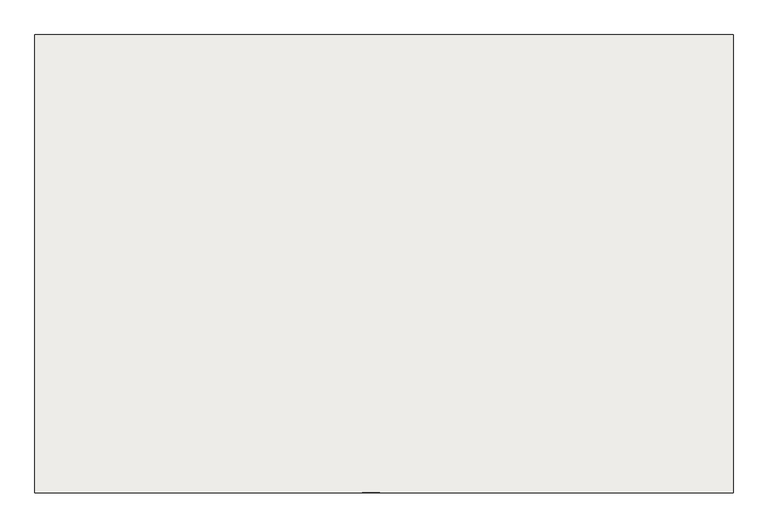
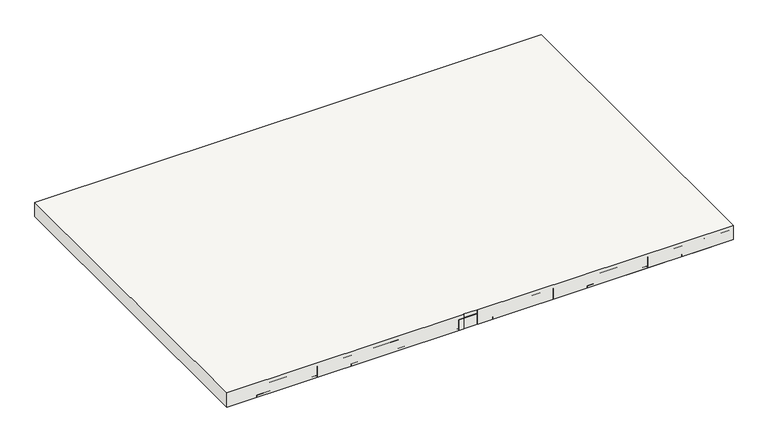
"""IFC4 building model written with IfcOpenShell, lengths in millimetres: slab geometry, Pano 2 (16 cm)."""

import ifcopenshell
import ifcopenshell.guid

model = None  # the IFC model being written
_history = None  # IfcOwnerHistory: only IFC2X3 demands one
_inside = {}  # id of a spatial element -> (the spatial element, [elements in it])
_under = {}  # id of a project, library or spatial element -> (it, [spatial elements below it])
_declared = {}  # id of a project -> (the project, [libraries it declares])
_typed = {}  # id of a type object -> (the type object, [elements of that type])
_made_of = {}  # id of a material, layer set ... -> (it, [elements and type objects made of it])


def new_model(schema):
    """Start an empty IFC model of exactly this schema.

    Asked for "IFC4X3", IfcOpenShell would pick the latest addendum, in which some entities
    have other attributes; the version numbers below select the first issue.
    IFC2X3 requires an IfcOwnerHistory on every rooted entity: one is made here for all.
    """
    global model, _history
    if schema == "IFC4X3":
        model = ifcopenshell.file(schema_version=(4, 3, 0, 0))
    else:
        model = ifcopenshell.file(schema=schema)
    _inside.clear()
    _under.clear()
    _declared.clear()
    _typed.clear()
    _made_of.clear()
    _history = None
    if model.schema == "IFC2X3":
        org = make("IfcOrganization", Name="unknown")
        user = make(
            "IfcPersonAndOrganization",
            ThePerson=make("IfcPerson", FamilyName="unknown"),
            TheOrganization=org,
        )
        app = make(
            "IfcApplication",
            ApplicationDeveloper=org,
            Version="unknown",
            ApplicationFullName="unknown",
            ApplicationIdentifier="unknown",
        )
        _history = make(
            "IfcOwnerHistory",
            OwningUser=user,
            OwningApplication=app,
            ChangeAction="ADDED",
            CreationDate=0,
        )
    return model


def make(cls, **values):
    """One entity of the class cls with the attributes given. An attribute that is None is left unset."""
    return model.create_entity(
        cls, **{name: value for name, value in values.items() if value is not None}
    )


def rooted(cls, **values):
    """An entity with a GlobalId (a new one), such as an element, a storey or a relation."""
    return make(cls, GlobalId=ifcopenshell.guid.new(), OwnerHistory=_history, **values)


def si_unit(unit_type, name, prefix=None):
    """IfcSIUnit, for example si_unit("LENGTHUNIT", "METRE", prefix="MILLI")."""
    return make("IfcSIUnit", UnitType=unit_type, Prefix=prefix, Name=name)


def assignment(units):
    """IfcUnitAssignment: the units of a project."""
    return None if units is None else make("IfcUnitAssignment", Units=units)


def point(xyz):
    """IfcCartesianPoint."""
    return None if xyz is None else make("IfcCartesianPoint", Coordinates=xyz)


def direction(xyz):
    """IfcDirection."""
    return None if xyz is None else make("IfcDirection", DirectionRatios=xyz)


def frame(location, z_axis=None, x_axis=None):
    """IfcAxis2Placement3D, a coordinate frame: its origin and axes. An axis left out is left unset."""
    return make(
        "IfcAxis2Placement3D",
        Location=point(location),
        Axis=direction(z_axis),
        RefDirection=direction(x_axis),
    )


def origin():
    """The frame at (0, 0, 0) with its axes left unset."""
    return frame((0.0, 0.0, 0.0))


def origin_with_axes():
    """The frame at (0, 0, 0) with the z axis (0, 0, 1) and the x axis (1, 0, 0) written out."""
    return frame((0.0, 0.0, 0.0), z_axis=(0.0, 0.0, 1.0), x_axis=(1.0, 0.0, 0.0))


def place(relative_to, where):
    """IfcLocalPlacement: puts the frame where relative to a parent placement (None: the world)."""
    return make(
        "IfcLocalPlacement", PlacementRelTo=relative_to, RelativePlacement=where
    )


def context(
    kind, dimensions, precision=None, world=None, true_north=None, identifier=None
):
    """IfcGeometricRepresentationContext, for example the 3D "Model" context."""
    return make(
        "IfcGeometricRepresentationContext",
        ContextIdentifier=identifier,
        ContextType=kind,
        CoordinateSpaceDimension=dimensions,
        Precision=precision,
        WorldCoordinateSystem=world,
        TrueNorth=true_north,
    )


def project(units=None, contexts=None):
    """IfcProject with its units and contexts."""
    return rooted(
        "IfcProject",
        Name="project",
        RepresentationContexts=contexts,
        UnitsInContext=assignment(units),
    )


def spatial(cls, under=None, at=None, **own):
    """A site, building, storey or space (cls), placed at a placement, below another one or the project."""
    s = rooted(cls, ObjectPlacement=at, **own)
    if under is not None:
        _under.setdefault(under.id(), (under, []))[1].append(s)
    return s


def polyline(points):
    """IfcPolyline through the points."""
    return make("IfcPolyline", Points=[point(p) for p in points])


def outline(outer, holes=None, kind="AREA"):
    """IfcArbitraryClosedProfileDef: a profile drawn as a closed curve; with holes, ...WithVoids."""
    if holes is None:
        return make("IfcArbitraryClosedProfileDef", ProfileType=kind, OuterCurve=outer)
    return make(
        "IfcArbitraryProfileDefWithVoids",
        ProfileType=kind,
        OuterCurve=outer,
        InnerCurves=holes,
    )


def extrude(swept, where, along, depth):
    """IfcExtrudedAreaSolid: the profile swept, set in the frame where, extruded along a direction by depth."""
    return make(
        "IfcExtrudedAreaSolid",
        SweptArea=swept,
        Position=where,
        ExtrudedDirection=direction(along),
        Depth=depth,
    )


def shape(context_of_items, identifier, shape_type, items):
    """IfcShapeRepresentation: the items that make up one representation, for example the "Body"."""
    return make(
        "IfcShapeRepresentation",
        ContextOfItems=context_of_items,
        RepresentationIdentifier=identifier,
        RepresentationType=shape_type,
        Items=items,
    )


def source(mapping_origin, context_of_items, identifier, shape_type, items):
    """IfcRepresentationMap: a shape defined once, which mapped items show again and again."""
    return make(
        "IfcRepresentationMap",
        MappingOrigin=mapping_origin,
        MappedRepresentation=shape(context_of_items, identifier, shape_type, items),
    )


def transform(
    local_origin,
    x_axis=None,
    y_axis=None,
    z_axis=None,
    scale=None,
    scale2=None,
    scale3=None,
    uniform=True,
):
    """IfcCartesianTransformationOperator3D, or its non-uniform kind. x_axis, y_axis, z_axis: its Axis1, 2, 3."""
    if uniform:
        return make(
            "IfcCartesianTransformationOperator3D",
            Axis1=direction(x_axis),
            Axis2=direction(y_axis),
            LocalOrigin=point(local_origin),
            Scale=scale,
            Axis3=direction(z_axis),
        )
    return make(
        "IfcCartesianTransformationOperator3DnonUniform",
        Axis1=direction(x_axis),
        Axis2=direction(y_axis),
        LocalOrigin=point(local_origin),
        Scale=scale,
        Axis3=direction(z_axis),
        Scale2=scale2,
        Scale3=scale3,
    )


def mapped(mapping_source, mapping_target):
    """IfcMappedItem: shows the shape of a source again, moved by a transform."""
    return make(
        "IfcMappedItem", MappingSource=mapping_source, MappingTarget=mapping_target
    )


def made_of(thing, what):
    """Note that an element or type object is made of a material, layer set ...; save() writes the relation."""
    if what is not None:
        _made_of.setdefault(what.id(), (what, []))[1].append(thing)
    return thing


def element(
    cls,
    number,
    at=None,
    inside=None,
    cuts=None,
    type_object=None,
    material=None,
    context=None,
    identifier="Body",
    shape_type=None,
    held_by="IfcProductDefinitionShape",
    body=None,
    shapes=None,
    **own,
):
    """One element of the class cls, such as IfcWall. Its Tag is "e" and its number.

    at: its placement. inside: the storey or other place that contains it. cuts: it is an
    opening in that element (IfcRelVoidsElement). A single representation is given by context,
    identifier, shape_type and body (its items); several are given by shapes. held_by: the class
    of the entity that holds the representations. save() writes the other relations.
    """
    e = rooted(cls, Tag="e%d" % number, ObjectPlacement=at, **own)
    if body is not None:
        shapes = [shape(context, identifier, shape_type, body)]
    if shapes is not None:
        e.Representation = make(held_by, Representations=shapes)
    if inside is not None:
        _inside.setdefault(inside.id(), (inside, []))[1].append(e)
    if cuts is not None:
        rooted(
            "IfcRelVoidsElement", RelatingBuildingElement=cuts, RelatedOpeningElement=e
        )
    if type_object is not None:
        _typed.setdefault(type_object.id(), (type_object, []))[1].append(e)
    return made_of(e, material)


def aggregate(whole, parts):
    """IfcRelAggregates: a whole, such as a stair, and the parts it consists of."""
    return rooted("IfcRelAggregates", RelatingObject=whole, RelatedObjects=parts)


def save(model, path):
    """Write the relations noted so far, then the file.

    IfcRelAggregates (storeys below a building ...), IfcRelContainedInSpatialStructure (elements
    in a storey), IfcRelDefinesByType, IfcRelAssociatesMaterial and IfcRelDeclares: one each for
    every whole, place, type object, material and project.
    """
    for whole, parts in _under.values():
        aggregate(whole, parts)
    for where, things in _inside.values():
        rooted(
            "IfcRelContainedInSpatialStructure",
            RelatedElements=things,
            RelatingStructure=where,
        )
    for kind, things in _typed.values():
        rooted("IfcRelDefinesByType", RelatedObjects=things, RelatingType=kind)
    for what, things in _made_of.values():
        rooted("IfcRelAssociatesMaterial", RelatedObjects=things, RelatingMaterial=what)
    for by, libraries in _declared.values():
        rooted("IfcRelDeclares", RelatingContext=by, RelatedDefinitions=libraries)
    model.write(path)


def slab_4fb4e0ab(model_context):
    return source(origin(), model_context, "Body", "SweptSolid", [
        extrude(outline(polyline([(-1000.0, 6010.0), (-1000.0, 2490.0), (-3710.0, 2490.0), (-3710.0, 2495.0), (-3850.0, 2495.0), (-3850.0, 2490.0), (-6360.0, 2490.0), (-6360.0, 6010.0), (-1000.0, 6010.0)])), origin_with_axes(), (0.0, 0.0, 1.0), 160.0),
        extrude(outline(polyline([(-5045.0, 5490.0), (-5405.0, 5490.0), (-5405.0, 5985.0), (-5045.0, 5985.0), (-5045.0, 5490.0)])), origin_with_axes(), (0.0, 0.0, 1.0), 120.0),
        extrude(outline(polyline([(-1545.0, 3990.0), (-1905.0, 3990.0), (-1905.0, 4485.0), (-1545.0, 4485.0), (-1545.0, 3990.0)])), origin_with_axes(), (0.0, 0.0, 1.0), 120.0),
        extrude(outline(polyline([(-4045.0, 4990.0), (-4405.0, 4990.0), (-4405.0, 5485.0), (-4045.0, 5485.0), (-4045.0, 4990.0)])), origin_with_axes(), (0.0, 0.0, 1.0), 120.0),
        extrude(outline(polyline([(-5545.0, 3490.0), (-5905.0, 3490.0), (-5905.0, 3985.0), (-5545.0, 3985.0), (-5545.0, 3490.0)])), origin_with_axes(), (0.0, 0.0, 1.0), 120.0),
        extrude(outline(polyline([(-2045.0, 5990.0), (-2405.0, 5990.0), (-2405.0, 6005.0), (-2045.0, 6005.0), (-2045.0, 5990.0)])), origin_with_axes(), (0.0, 0.0, 1.0), 120.0),
        extrude(outline(polyline([(-3545.0, 2490.0), (-3905.0, 2490.0), (-3905.0, 2985.0), (-3545.0, 2985.0), (-3545.0, 2490.0)])), origin_with_axes(), (0.0, 0.0, 1.0), 120.0),
        extrude(outline(polyline([(-5545.0, 2990.0), (-5905.0, 2990.0), (-5905.0, 3485.0), (-5545.0, 3485.0), (-5545.0, 2990.0)])), origin_with_axes(), (0.0, 0.0, 1.0), 120.0),
        extrude(outline(polyline([(-3905.0, 2490.0), (-4045.0, 2490.0), (-4045.0, 6010.0), (-3905.0, 6010.0), (-3905.0, 2490.0)])), origin_with_axes(), (0.0, 0.0, 1.0), 24.0),
        extrude(outline(polyline([(-5545.0, 5490.0), (-5905.0, 5490.0), (-5905.0, 5985.0), (-5545.0, 5985.0), (-5545.0, 5490.0)])), origin_with_axes(), (0.0, 0.0, 1.0), 120.0),
        extrude(outline(polyline([(-2545.0, 2990.0), (-2905.0, 2990.0), (-2905.0, 3485.0), (-2545.0, 3485.0), (-2545.0, 2990.0)])), origin_with_axes(), (0.0, 0.0, 1.0), 120.0),
        extrude(outline(polyline([(-3045.0, 5490.0), (-3405.0, 5490.0), (-3405.0, 5985.0), (-3045.0, 5985.0), (-3045.0, 5490.0)])), origin_with_axes(), (0.0, 0.0, 1.0), 120.0),
        extrude(outline(polyline([(-2045.0, 2490.0), (-2405.0, 2490.0), (-2405.0, 2985.0), (-2045.0, 2985.0), (-2045.0, 2490.0)])), origin_with_axes(), (0.0, 0.0, 1.0), 120.0),
        extrude(outline(polyline([(-4045.0, 5490.0), (-4405.0, 5490.0), (-4405.0, 5985.0), (-4045.0, 5985.0), (-4045.0, 5490.0)])), origin_with_axes(), (0.0, 0.0, 1.0), 120.0),
        extrude(outline(polyline([(-2545.0, 3490.0), (-2905.0, 3490.0), (-2905.0, 3985.0), (-2545.0, 3985.0), (-2545.0, 3490.0)])), origin_with_axes(), (0.0, 0.0, 1.0), 120.0),
        extrude(outline(polyline([(-2545.0, 2490.0), (-2905.0, 2490.0), (-2905.0, 2985.0), (-2545.0, 2985.0), (-2545.0, 2490.0)])), origin_with_axes(), (0.0, 0.0, 1.0), 120.0),
        extrude(outline(polyline([(-2545.0, 4990.0), (-2905.0, 4990.0), (-2905.0, 5485.0), (-2545.0, 5485.0), (-2545.0, 4990.0)])), origin_with_axes(), (0.0, 0.0, 1.0), 120.0),
        extrude(outline(polyline([(-3045.0, 2490.0), (-3405.0, 2490.0), (-3405.0, 2985.0), (-3045.0, 2985.0), (-3045.0, 2490.0)])), origin_with_axes(), (0.0, 0.0, 1.0), 120.0),
        extrude(outline(polyline([(-1044.5, 4990.0), (-1404.5, 4990.0), (-1404.5, 5485.0), (-1044.5, 5485.0), (-1044.5, 4990.0)])), origin_with_axes(), (0.0, 0.0, 1.0), 120.0),
        extrude(outline(polyline([(-4045.0, 2490.0), (-4405.0, 2490.0), (-4405.0, 2985.0), (-4045.0, 2985.0), (-4045.0, 2490.0)])), origin_with_axes(), (0.0, 0.0, 1.0), 120.0),
        extrude(outline(polyline([(-1545.0, 2490.0), (-1905.0, 2490.0), (-1905.0, 2985.0), (-1545.0, 2985.0), (-1545.0, 2490.0)])), origin_with_axes(), (0.0, 0.0, 1.0), 120.0),
        extrude(outline(polyline([(-2045.0, 3490.0), (-2405.0, 3490.0), (-2405.0, 3985.0), (-2045.0, 3985.0), (-2045.0, 3490.0)])), origin_with_axes(), (0.0, 0.0, 1.0), 120.0),
        extrude(outline(polyline([(-5545.0, 2490.0), (-5905.0, 2490.0), (-5905.0, 2985.0), (-5545.0, 2985.0), (-5545.0, 2490.0)])), origin_with_axes(), (0.0, 0.0, 1.0), 120.0),
        extrude(outline(polyline([(-2045.0, 5490.0), (-2405.0, 5490.0), (-2405.0, 5985.0), (-2045.0, 5985.0), (-2045.0, 5490.0)])), origin_with_axes(), (0.0, 0.0, 1.0), 120.0),
        extrude(outline(polyline([(-4545.0, 5490.0), (-4905.0, 5490.0), (-4905.0, 5985.0), (-4545.0, 5985.0), (-4545.0, 5490.0)])), origin_with_axes(), (0.0, 0.0, 1.0), 120.0),
        extrude(outline(polyline([(-2045.0, 4990.0), (-2405.0, 4990.0), (-2405.0, 5485.0), (-2045.0, 5485.0), (-2045.0, 4990.0)])), origin_with_axes(), (0.0, 0.0, 1.0), 120.0),
        extrude(outline(polyline([(-4045.0, 4490.0), (-4405.0, 4490.0), (-4405.0, 4985.0), (-4045.0, 4985.0), (-4045.0, 4490.0)])), origin_with_axes(), (0.0, 0.0, 1.0), 120.0),
        extrude(outline(polyline([(-5545.0, 3990.0), (-5905.0, 3990.0), (-5905.0, 4485.0), (-5545.0, 4485.0), (-5545.0, 3990.0)])), origin_with_axes(), (0.0, 0.0, 1.0), 120.0),
        extrude(outline(polyline([(-3045.0, 3490.0), (-3405.0, 3490.0), (-3405.0, 3985.0), (-3045.0, 3985.0), (-3045.0, 3490.0)])), origin_with_axes(), (0.0, 0.0, 1.0), 120.0),
        extrude(outline(polyline([(-3045.0, 5990.0), (-3405.0, 5990.0), (-3405.0, 6005.0), (-3045.0, 6005.0), (-3045.0, 5990.0)])), origin_with_axes(), (0.0, 0.0, 1.0), 120.0),
        extrude(outline(polyline([(-4545.0, 3490.0), (-4905.0, 3490.0), (-4905.0, 3985.0), (-4545.0, 3985.0), (-4545.0, 3490.0)])), origin_with_axes(), (0.0, 0.0, 1.0), 120.0),
        extrude(outline(polyline([(-4545.0, 5990.0), (-4905.0, 5990.0), (-4905.0, 6005.0), (-4545.0, 6005.0), (-4545.0, 5990.0)])), origin_with_axes(), (0.0, 0.0, 1.0), 120.0),
        extrude(outline(polyline([(-3045.0, 4490.0), (-3405.0, 4490.0), (-3405.0, 4985.0), (-3045.0, 4985.0), (-3045.0, 4490.0)])), origin_with_axes(), (0.0, 0.0, 1.0), 120.0),
        extrude(outline(polyline([(-4045.0, 2990.0), (-4405.0, 2990.0), (-4405.0, 3485.0), (-4045.0, 3485.0), (-4045.0, 2990.0)])), origin_with_axes(), (0.0, 0.0, 1.0), 120.0),
        extrude(outline(polyline([(-4545.0, 2490.0), (-4905.0, 2490.0), (-4905.0, 2985.0), (-4545.0, 2985.0), (-4545.0, 2490.0)])), origin_with_axes(), (0.0, 0.0, 1.0), 120.0),
        extrude(outline(polyline([(-2045.0, 3990.0), (-2405.0, 3990.0), (-2405.0, 4485.0), (-2045.0, 4485.0), (-2045.0, 3990.0)])), origin_with_axes(), (0.0, 0.0, 1.0), 120.0),
        extrude(outline(polyline([(-5045.0, 5990.0), (-5405.0, 5990.0), (-5405.0, 6005.0), (-5045.0, 6005.0), (-5045.0, 5990.0)])), origin_with_axes(), (0.0, 0.0, 1.0), 120.0),
        extrude(outline(polyline([(-2045.0, 2990.0), (-2405.0, 2990.0), (-2405.0, 3485.0), (-2045.0, 3485.0), (-2045.0, 2990.0)])), origin_with_axes(), (0.0, 0.0, 1.0), 120.0),
        extrude(outline(polyline([(-2545.0, 5990.0), (-2905.0, 5990.0), (-2905.0, 6005.0), (-2545.0, 6005.0), (-2545.0, 5990.0)])), origin_with_axes(), (0.0, 0.0, 1.0), 120.0),
        extrude(outline(polyline([(-1545.0, 4990.0), (-1905.0, 4990.0), (-1905.0, 5485.0), (-1545.0, 5485.0), (-1545.0, 4990.0)])), origin_with_axes(), (0.0, 0.0, 1.0), 120.0),
        extrude(outline(polyline([(-4045.0, 5990.0), (-4405.0, 5990.0), (-4405.0, 6005.0), (-4045.0, 6005.0), (-4045.0, 5990.0)])), origin_with_axes(), (0.0, 0.0, 1.0), 120.0),
        extrude(outline(polyline([(-2045.0, 4490.0), (-2405.0, 4490.0), (-2405.0, 4985.0), (-2045.0, 4985.0), (-2045.0, 4490.0)])), origin_with_axes(), (0.0, 0.0, 1.0), 120.0),
        extrude(outline(polyline([(-4905.0, 2490.0), (-5045.0, 2490.0), (-5045.0, 6010.0), (-4905.0, 6010.0), (-4905.0, 2490.0)])), origin_with_axes(), (0.0, 0.0, 1.0), 24.0),
        extrude(outline(polyline([(-3045.0, 3990.0), (-3405.0, 3990.0), (-3405.0, 4485.0), (-3045.0, 4485.0), (-3045.0, 3990.0)])), origin_with_axes(), (0.0, 0.0, 1.0), 120.0),
        extrude(outline(polyline([(-1545.0, 5990.0), (-1905.0, 5990.0), (-1905.0, 6005.0), (-1545.0, 6005.0), (-1545.0, 5990.0)])), origin_with_axes(), (0.0, 0.0, 1.0), 120.0),
        extrude(outline(polyline([(-3405.0, 2490.0), (-3545.0, 2490.0), (-3545.0, 6010.0), (-3405.0, 6010.0), (-3405.0, 2490.0)])), origin_with_axes(), (0.0, 0.0, 1.0), 24.0),
        extrude(outline(polyline([(-2545.0, 5490.0), (-2905.0, 5490.0), (-2905.0, 5985.0), (-2545.0, 5985.0), (-2545.0, 5490.0)])), origin_with_axes(), (0.0, 0.0, 1.0), 120.0),
        extrude(outline(polyline([(-4545.0, 2990.0), (-4905.0, 2990.0), (-4905.0, 3485.0), (-4545.0, 3485.0), (-4545.0, 2990.0)])), origin_with_axes(), (0.0, 0.0, 1.0), 120.0),
        extrude(outline(polyline([(-4045.0, 3990.0), (-4405.0, 3990.0), (-4405.0, 4485.0), (-4045.0, 4485.0), (-4045.0, 3990.0)])), origin_with_axes(), (0.0, 0.0, 1.0), 120.0),
        extrude(outline(polyline([(-3545.0, 3990.0), (-3905.0, 3990.0), (-3905.0, 4485.0), (-3545.0, 4485.0), (-3545.0, 3990.0)])), origin_with_axes(), (0.0, 0.0, 1.0), 120.0),
        extrude(outline(polyline([(-1545.0, 5490.0), (-1905.0, 5490.0), (-1905.0, 5985.0), (-1545.0, 5985.0), (-1545.0, 5490.0)])), origin_with_axes(), (0.0, 0.0, 1.0), 120.0),
        extrude(outline(polyline([(-5045.0, 4990.0), (-5405.0, 4990.0), (-5405.0, 5485.0), (-5045.0, 5485.0), (-5045.0, 4990.0)])), origin_with_axes(), (0.0, 0.0, 1.0), 120.0),
        extrude(outline(polyline([(-1545.0, 4490.0), (-1905.0, 4490.0), (-1905.0, 4985.0), (-1545.0, 4985.0), (-1545.0, 4490.0)])), origin_with_axes(), (0.0, 0.0, 1.0), 120.0),
        extrude(outline(polyline([(-2545.0, 4490.0), (-2905.0, 4490.0), (-2905.0, 4985.0), (-2545.0, 4985.0), (-2545.0, 4490.0)])), origin_with_axes(), (0.0, 0.0, 1.0), 120.0),
        extrude(outline(polyline([(-5405.0, 2490.0), (-5545.0, 2490.0), (-5545.0, 6010.0), (-5405.0, 6010.0), (-5405.0, 2490.0)])), origin_with_axes(), (0.0, 0.0, 1.0), 24.0),
        extrude(outline(polyline([(-5545.0, 4990.0), (-5905.0, 4990.0), (-5905.0, 5485.0), (-5545.0, 5485.0), (-5545.0, 4990.0)])), origin_with_axes(), (0.0, 0.0, 1.0), 120.0),
        extrude(outline(polyline([(-5045.0, 3490.0), (-5405.0, 3490.0), (-5405.0, 3985.0), (-5045.0, 3985.0), (-5045.0, 3490.0)])), origin_with_axes(), (0.0, 0.0, 1.0), 120.0),
        extrude(outline(polyline([(-3545.0, 5490.0), (-3905.0, 5490.0), (-3905.0, 5985.0), (-3545.0, 5985.0), (-3545.0, 5490.0)])), origin_with_axes(), (0.0, 0.0, 1.0), 120.0),
        extrude(outline(polyline([(-4045.0, 3490.0), (-4405.0, 3490.0), (-4405.0, 3985.0), (-4045.0, 3985.0), (-4045.0, 3490.0)])), origin_with_axes(), (0.0, 0.0, 1.0), 120.0),
        extrude(outline(polyline([(-5905.0, 2490.0), (-6045.0, 2490.0), (-6045.0, 6010.0), (-5905.0, 6010.0), (-5905.0, 2490.0)])), origin_with_axes(), (0.0, 0.0, 1.0), 24.0),
        extrude(outline(polyline([(-5545.0, 4490.0), (-5905.0, 4490.0), (-5905.0, 4985.0), (-5545.0, 4985.0), (-5545.0, 4490.0)])), origin_with_axes(), (0.0, 0.0, 1.0), 120.0),
        extrude(outline(polyline([(-1044.5, 4490.0), (-1404.5, 4490.0), (-1404.5, 4985.0), (-1044.5, 4985.0), (-1044.5, 4490.0)])), origin_with_axes(), (0.0, 0.0, 1.0), 120.0),
        extrude(outline(polyline([(-4405.0, 2490.0), (-4545.0, 2490.0), (-4545.0, 6010.0), (-4405.0, 6010.0), (-4405.0, 2490.0)])), origin_with_axes(), (0.0, 0.0, 1.0), 24.0),
        extrude(outline(polyline([(-1044.5, 5490.0), (-1404.5, 5490.0), (-1404.5, 5985.0), (-1044.5, 5985.0), (-1044.5, 5490.0)])), origin_with_axes(), (0.0, 0.0, 1.0), 120.0),
        extrude(outline(polyline([(-5045.0, 2990.0), (-5405.0, 2990.0), (-5405.0, 3485.0), (-5045.0, 3485.0), (-5045.0, 2990.0)])), origin_with_axes(), (0.0, 0.0, 1.0), 120.0),
        extrude(outline(polyline([(-5045.0, 4490.0), (-5405.0, 4490.0), (-5405.0, 4985.0), (-5045.0, 4985.0), (-5045.0, 4490.0)])), origin_with_axes(), (0.0, 0.0, 1.0), 120.0),
        extrude(outline(polyline([(-5045.0, 2490.0), (-5405.0, 2490.0), (-5405.0, 2985.0), (-5045.0, 2985.0), (-5045.0, 2490.0)])), origin_with_axes(), (0.0, 0.0, 1.0), 120.0),
        extrude(outline(polyline([(-3545.0, 3490.0), (-3905.0, 3490.0), (-3905.0, 3985.0), (-3545.0, 3985.0), (-3545.0, 3490.0)])), origin_with_axes(), (0.0, 0.0, 1.0), 120.0),
        extrude(outline(polyline([(-4545.0, 3990.0), (-4905.0, 3990.0), (-4905.0, 4485.0), (-4545.0, 4485.0), (-4545.0, 3990.0)])), origin_with_axes(), (0.0, 0.0, 1.0), 120.0),
        extrude(outline(polyline([(-1545.0, 2990.0), (-1905.0, 2990.0), (-1905.0, 3485.0), (-1545.0, 3485.0), (-1545.0, 2990.0)])), origin_with_axes(), (0.0, 0.0, 1.0), 120.0),
        extrude(outline(polyline([(-1405.0, 2490.0), (-1545.0, 2490.0), (-1545.0, 6010.0), (-1405.0, 6010.0), (-1405.0, 2490.0)])), origin_with_axes(), (0.0, 0.0, 1.0), 24.0),
        extrude(outline(polyline([(-3045.0, 4990.0), (-3405.0, 4990.0), (-3405.0, 5485.0), (-3045.0, 5485.0), (-3045.0, 4990.0)])), origin_with_axes(), (0.0, 0.0, 1.0), 120.0),
        extrude(outline(polyline([(-1545.0, 3490.0), (-1905.0, 3490.0), (-1905.0, 3985.0), (-1545.0, 3985.0), (-1545.0, 3490.0)])), origin_with_axes(), (0.0, 0.0, 1.0), 120.0),
        extrude(outline(polyline([(-4545.0, 4490.0), (-4905.0, 4490.0), (-4905.0, 4985.0), (-4545.0, 4985.0), (-4545.0, 4490.0)])), origin_with_axes(), (0.0, 0.0, 1.0), 120.0),
        extrude(outline(polyline([(-3545.0, 4490.0), (-3905.0, 4490.0), (-3905.0, 4985.0), (-3545.0, 4985.0), (-3545.0, 4490.0)])), origin_with_axes(), (0.0, 0.0, 1.0), 120.0),
        extrude(outline(polyline([(-1044.5, 3490.0), (-1404.5, 3490.0), (-1404.5, 3985.0), (-1044.5, 3985.0), (-1044.5, 3490.0)])), origin_with_axes(), (0.0, 0.0, 1.0), 120.0),
        extrude(outline(polyline([(-1044.5, 2490.0), (-1404.5, 2490.0), (-1404.5, 2985.0), (-1044.5, 2985.0), (-1044.5, 2490.0)])), origin_with_axes(), (0.0, 0.0, 1.0), 120.0),
        extrude(outline(polyline([(-3545.0, 5990.0), (-3905.0, 5990.0), (-3905.0, 6005.0), (-3545.0, 6005.0), (-3545.0, 5990.0)])), origin_with_axes(), (0.0, 0.0, 1.0), 120.0),
        extrude(outline(polyline([(-3545.0, 2990.0), (-3905.0, 2990.0), (-3905.0, 3485.0), (-3545.0, 3485.0), (-3545.0, 2990.0)])), origin_with_axes(), (0.0, 0.0, 1.0), 120.0),
        extrude(outline(polyline([(-5045.0, 3990.0), (-5405.0, 3990.0), (-5405.0, 4485.0), (-5045.0, 4485.0), (-5045.0, 3990.0)])), origin_with_axes(), (0.0, 0.0, 1.0), 120.0),
        extrude(outline(polyline([(-1044.5, 2990.0), (-1404.5, 2990.0), (-1404.5, 3485.0), (-1044.5, 3485.0), (-1044.5, 2990.0)])), origin_with_axes(), (0.0, 0.0, 1.0), 120.0),
        extrude(outline(polyline([(-5545.0, 5990.0), (-5905.0, 5990.0), (-5905.0, 6005.0), (-5545.0, 6005.0), (-5545.0, 5990.0)])), origin_with_axes(), (0.0, 0.0, 1.0), 120.0),
        extrude(outline(polyline([(-1905.0, 2490.0), (-2045.0, 2490.0), (-2045.0, 6010.0), (-1905.0, 6010.0), (-1905.0, 2490.0)])), origin_with_axes(), (0.0, 0.0, 1.0), 24.0),
        extrude(outline(polyline([(-3045.0, 2990.0), (-3405.0, 2990.0), (-3405.0, 3485.0), (-3045.0, 3485.0), (-3045.0, 2990.0)])), origin_with_axes(), (0.0, 0.0, 1.0), 120.0),
        extrude(outline(polyline([(-2905.0, 2490.0), (-3045.0, 2490.0), (-3045.0, 6010.0), (-2905.0, 6010.0), (-2905.0, 2490.0)])), origin_with_axes(), (0.0, 0.0, 1.0), 24.0),
        extrude(outline(polyline([(-1044.5, 3990.0), (-1404.5, 3990.0), (-1404.5, 4485.0), (-1044.5, 4485.0), (-1044.5, 3990.0)])), origin_with_axes(), (0.0, 0.0, 1.0), 120.0),
        extrude(outline(polyline([(-2405.0, 2490.0), (-2545.0, 2490.0), (-2545.0, 6010.0), (-2405.0, 6010.0), (-2405.0, 2490.0)])), origin_with_axes(), (0.0, 0.0, 1.0), 24.0),
        extrude(outline(polyline([(-2545.0, 3990.0), (-2905.0, 3990.0), (-2905.0, 4485.0), (-2545.0, 4485.0), (-2545.0, 3990.0)])), origin_with_axes(), (0.0, 0.0, 1.0), 120.0),
        extrude(outline(polyline([(-1044.5, 5990.0), (-1404.5, 5990.0), (-1404.5, 6005.0), (-1044.5, 6005.0), (-1044.5, 5990.0)])), origin_with_axes(), (0.0, 0.0, 1.0), 120.0),
        extrude(outline(polyline([(-4545.0, 4990.0), (-4905.0, 4990.0), (-4905.0, 5485.0), (-4545.0, 5485.0), (-4545.0, 4990.0)])), origin_with_axes(), (0.0, 0.0, 1.0), 120.0),
        extrude(outline(polyline([(-3545.0, 4990.0), (-3905.0, 4990.0), (-3905.0, 5485.0), (-3545.0, 5485.0), (-3545.0, 4990.0)])), origin_with_axes(), (0.0, 0.0, 1.0), 120.0),
    ])


if __name__ == "__main__":
    model = new_model("IFC4")
    model_context = context("Model", 3, world=origin())
    ifc_project = project(units=[si_unit("LENGTHUNIT", "METRE", prefix="MILLI")], contexts=[model_context])
    site = spatial("IfcSite", under=ifc_project)
    building = spatial("IfcBuilding", under=site)
    placement = place(None, origin())
    slab_shape = slab_4fb4e0ab(model_context)
    element("IfcSlab", 1, ObjectType="Pano 2 (16 cm)", at=placement, inside=building, context=model_context, shape_type="MappedRepresentation", body=[
        mapped(slab_shape, transform((0.0, 0.0, 0.0), x_axis=(1.0, 0.0, 0.0), y_axis=(0.0, 1.0, 0.0), z_axis=(0.0, 0.0, 1.0))),
    ])
    save(model, "model.ifc")

# Revit data of these elements
# Element 1 (IfcSlab, "Pano 2 (16 cm)")
#   Materials on its faces: "Molde de poliestireno", "Concreto armado", "RGB 168-169-158"
# Materials
#   "Molde de poliestireno": class "Não atribuído", colour RGB 255 255 255, transparency 0
#   "Concreto armado": class "Não atribuído", colour RGB 168 169 158, transparency 0
#   "RGB 168-169-158": class "Não atribuído", colour RGB 168 169 158, transparency 0
